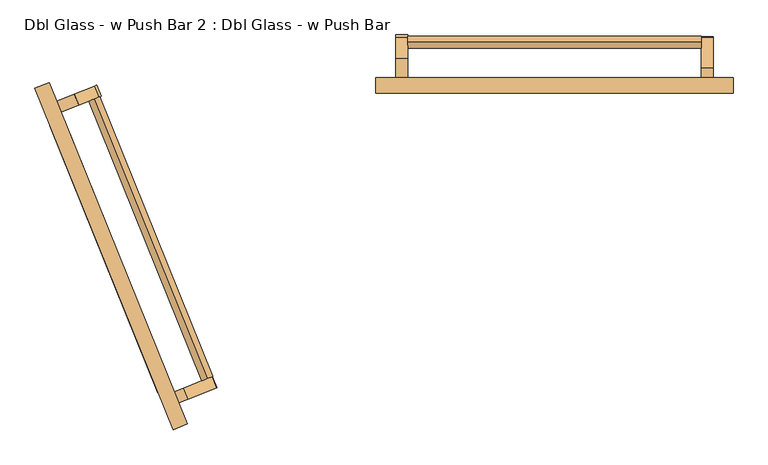
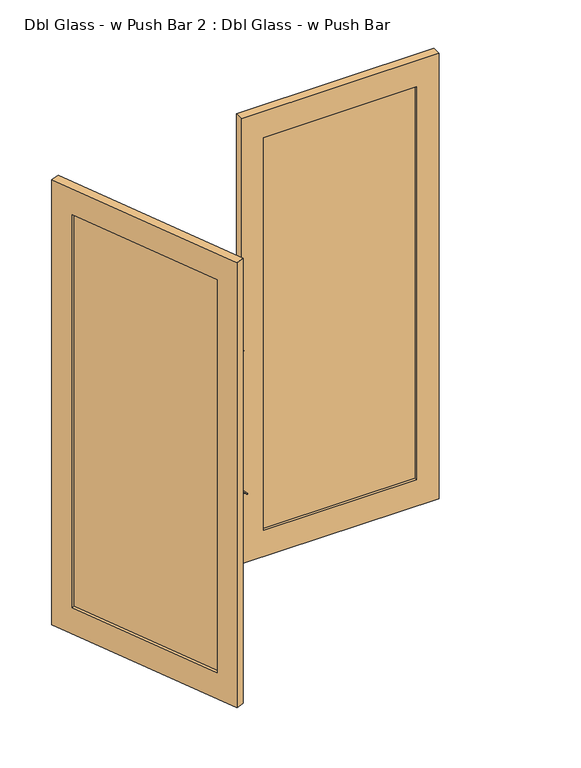
"""IFC4 building model written with IfcOpenShell, lengths in millimetres: door geometry, Dbl Glass - w Push Bar 2 : Dbl Glass - w Push Bar."""

import ifcopenshell
import ifcopenshell.guid

model = None  # the IFC model being written
_history = None  # IfcOwnerHistory: only IFC2X3 demands one
_inside = {}  # id of a spatial element -> (the spatial element, [elements in it])
_under = {}  # id of a project, library or spatial element -> (it, [spatial elements below it])
_declared = {}  # id of a project -> (the project, [libraries it declares])
_typed = {}  # id of a type object -> (the type object, [elements of that type])
_made_of = {}  # id of a material, layer set ... -> (it, [elements and type objects made of it])


def new_model(schema):
    """Start an empty IFC model of exactly this schema.

    Asked for "IFC4X3", IfcOpenShell would pick the latest addendum, in which some entities
    have other attributes; the version numbers below select the first issue.
    IFC2X3 requires an IfcOwnerHistory on every rooted entity: one is made here for all.
    """
    global model, _history
    if schema == "IFC4X3":
        model = ifcopenshell.file(schema_version=(4, 3, 0, 0))
    else:
        model = ifcopenshell.file(schema=schema)
    _inside.clear()
    _under.clear()
    _declared.clear()
    _typed.clear()
    _made_of.clear()
    _history = None
    if model.schema == "IFC2X3":
        org = make("IfcOrganization", Name="unknown")
        user = make(
            "IfcPersonAndOrganization",
            ThePerson=make("IfcPerson", FamilyName="unknown"),
            TheOrganization=org,
        )
        app = make(
            "IfcApplication",
            ApplicationDeveloper=org,
            Version="unknown",
            ApplicationFullName="unknown",
            ApplicationIdentifier="unknown",
        )
        _history = make(
            "IfcOwnerHistory",
            OwningUser=user,
            OwningApplication=app,
            ChangeAction="ADDED",
            CreationDate=0,
        )
    return model


def make(cls, **values):
    """One entity of the class cls with the attributes given. An attribute that is None is left unset."""
    return model.create_entity(
        cls, **{name: value for name, value in values.items() if value is not None}
    )


def rooted(cls, **values):
    """An entity with a GlobalId (a new one), such as an element, a storey or a relation."""
    return make(cls, GlobalId=ifcopenshell.guid.new(), OwnerHistory=_history, **values)


def si_unit(unit_type, name, prefix=None):
    """IfcSIUnit, for example si_unit("LENGTHUNIT", "METRE", prefix="MILLI")."""
    return make("IfcSIUnit", UnitType=unit_type, Prefix=prefix, Name=name)


def assignment(units):
    """IfcUnitAssignment: the units of a project."""
    return None if units is None else make("IfcUnitAssignment", Units=units)


def point(xyz):
    """IfcCartesianPoint."""
    return None if xyz is None else make("IfcCartesianPoint", Coordinates=xyz)


def direction(xyz):
    """IfcDirection."""
    return None if xyz is None else make("IfcDirection", DirectionRatios=xyz)


def frame(location, z_axis=None, x_axis=None):
    """IfcAxis2Placement3D, a coordinate frame: its origin and axes. An axis left out is left unset."""
    return make(
        "IfcAxis2Placement3D",
        Location=point(location),
        Axis=direction(z_axis),
        RefDirection=direction(x_axis),
    )


def frame_2d(location, x_axis=None):
    """IfcAxis2Placement2D, a coordinate frame in the plane: its origin and x axis."""
    return make(
        "IfcAxis2Placement2D", Location=point(location), RefDirection=direction(x_axis)
    )


def origin():
    """The frame at (0, 0, 0) with its axes left unset."""
    return frame((0.0, 0.0, 0.0))


def place(relative_to, where):
    """IfcLocalPlacement: puts the frame where relative to a parent placement (None: the world)."""
    return make(
        "IfcLocalPlacement", PlacementRelTo=relative_to, RelativePlacement=where
    )


def context(
    kind, dimensions, precision=None, world=None, true_north=None, identifier=None
):
    """IfcGeometricRepresentationContext, for example the 3D "Model" context."""
    return make(
        "IfcGeometricRepresentationContext",
        ContextIdentifier=identifier,
        ContextType=kind,
        CoordinateSpaceDimension=dimensions,
        Precision=precision,
        WorldCoordinateSystem=world,
        TrueNorth=true_north,
    )


def project(units=None, contexts=None):
    """IfcProject with its units and contexts."""
    return rooted(
        "IfcProject",
        Name="project",
        RepresentationContexts=contexts,
        UnitsInContext=assignment(units),
    )


def spatial(cls, under=None, at=None, **own):
    """A site, building, storey or space (cls), placed at a placement, below another one or the project."""
    s = rooted(cls, ObjectPlacement=at, **own)
    if under is not None:
        _under.setdefault(under.id(), (under, []))[1].append(s)
    return s


def polyline(points):
    """IfcPolyline through the points."""
    return make("IfcPolyline", Points=[point(p) for p in points])


def circle_curve(where, radius):
    """IfcCircle in the frame where."""
    return make("IfcCircle", Position=where, Radius=radius)


def trimmed(basis, trim1, trim2, sense, master):
    """IfcTrimmedCurve: the piece of a basis curve between two trims."""
    return make(
        "IfcTrimmedCurve",
        BasisCurve=basis,
        Trim1=trim1,
        Trim2=trim2,
        SenseAgreement=sense,
        MasterRepresentation=master,
    )


def segment(curve, same_sense, transition):
    """IfcCompositeCurveSegment."""
    return make(
        "IfcCompositeCurveSegment",
        Transition=transition,
        SameSense=same_sense,
        ParentCurve=curve,
    )


def composite_curve(segments, self_intersect=None):
    """IfcCompositeCurve: segments joined end to end."""
    return make("IfcCompositeCurve", Segments=segments, SelfIntersect=self_intersect)


def outline(outer, holes=None, kind="AREA"):
    """IfcArbitraryClosedProfileDef: a profile drawn as a closed curve; with holes, ...WithVoids."""
    if holes is None:
        return make("IfcArbitraryClosedProfileDef", ProfileType=kind, OuterCurve=outer)
    return make(
        "IfcArbitraryProfileDefWithVoids",
        ProfileType=kind,
        OuterCurve=outer,
        InnerCurves=holes,
    )


def extrude(swept, where, along, depth):
    """IfcExtrudedAreaSolid: the profile swept, set in the frame where, extruded along a direction by depth."""
    return make(
        "IfcExtrudedAreaSolid",
        SweptArea=swept,
        Position=where,
        ExtrudedDirection=direction(along),
        Depth=depth,
    )


def shape(context_of_items, identifier, shape_type, items):
    """IfcShapeRepresentation: the items that make up one representation, for example the "Body"."""
    return make(
        "IfcShapeRepresentation",
        ContextOfItems=context_of_items,
        RepresentationIdentifier=identifier,
        RepresentationType=shape_type,
        Items=items,
    )


def source(mapping_origin, context_of_items, identifier, shape_type, items):
    """IfcRepresentationMap: a shape defined once, which mapped items show again and again."""
    return make(
        "IfcRepresentationMap",
        MappingOrigin=mapping_origin,
        MappedRepresentation=shape(context_of_items, identifier, shape_type, items),
    )


def transform(
    local_origin,
    x_axis=None,
    y_axis=None,
    z_axis=None,
    scale=None,
    scale2=None,
    scale3=None,
    uniform=True,
):
    """IfcCartesianTransformationOperator3D, or its non-uniform kind. x_axis, y_axis, z_axis: its Axis1, 2, 3."""
    if uniform:
        return make(
            "IfcCartesianTransformationOperator3D",
            Axis1=direction(x_axis),
            Axis2=direction(y_axis),
            LocalOrigin=point(local_origin),
            Scale=scale,
            Axis3=direction(z_axis),
        )
    return make(
        "IfcCartesianTransformationOperator3DnonUniform",
        Axis1=direction(x_axis),
        Axis2=direction(y_axis),
        LocalOrigin=point(local_origin),
        Scale=scale,
        Axis3=direction(z_axis),
        Scale2=scale2,
        Scale3=scale3,
    )


def mapped(mapping_source, mapping_target):
    """IfcMappedItem: shows the shape of a source again, moved by a transform."""
    return make(
        "IfcMappedItem", MappingSource=mapping_source, MappingTarget=mapping_target
    )


def made_of(thing, what):
    """Note that an element or type object is made of a material, layer set ...; save() writes the relation."""
    if what is not None:
        _made_of.setdefault(what.id(), (what, []))[1].append(thing)
    return thing


def element(
    cls,
    number,
    at=None,
    inside=None,
    cuts=None,
    type_object=None,
    material=None,
    context=None,
    identifier="Body",
    shape_type=None,
    held_by="IfcProductDefinitionShape",
    body=None,
    shapes=None,
    **own,
):
    """One element of the class cls, such as IfcWall. Its Tag is "e" and its number.

    at: its placement. inside: the storey or other place that contains it. cuts: it is an
    opening in that element (IfcRelVoidsElement). A single representation is given by context,
    identifier, shape_type and body (its items); several are given by shapes. held_by: the class
    of the entity that holds the representations. save() writes the other relations.
    """
    e = rooted(cls, Tag="e%d" % number, ObjectPlacement=at, **own)
    if body is not None:
        shapes = [shape(context, identifier, shape_type, body)]
    if shapes is not None:
        e.Representation = make(held_by, Representations=shapes)
    if inside is not None:
        _inside.setdefault(inside.id(), (inside, []))[1].append(e)
    if cuts is not None:
        rooted(
            "IfcRelVoidsElement", RelatingBuildingElement=cuts, RelatedOpeningElement=e
        )
    if type_object is not None:
        _typed.setdefault(type_object.id(), (type_object, []))[1].append(e)
    return made_of(e, material)


def aggregate(whole, parts):
    """IfcRelAggregates: a whole, such as a stair, and the parts it consists of."""
    return rooted("IfcRelAggregates", RelatingObject=whole, RelatedObjects=parts)


def save(model, path):
    """Write the relations noted so far, then the file.

    IfcRelAggregates (storeys below a building ...), IfcRelContainedInSpatialStructure (elements
    in a storey), IfcRelDefinesByType, IfcRelAssociatesMaterial and IfcRelDeclares: one each for
    every whole, place, type object, material and project.
    """
    for whole, parts in _under.values():
        aggregate(whole, parts)
    for where, things in _inside.values():
        rooted(
            "IfcRelContainedInSpatialStructure",
            RelatedElements=things,
            RelatingStructure=where,
        )
    for kind, things in _typed.values():
        rooted("IfcRelDefinesByType", RelatedObjects=things, RelatingType=kind)
    for what, things in _made_of.values():
        rooted("IfcRelAssociatesMaterial", RelatedObjects=things, RelatingMaterial=what)
    for by, libraries in _declared.values():
        rooted("IfcRelDeclares", RelatingContext=by, RelatedDefinitions=libraries)
    model.write(path)


def dbl_glass_w_push_bar_2_dbl_glass_w_push_bar_dfafdb44(model_context):
    return source(origin(), model_context, "Body", "SweptSolid", [
        extrude(outline(composite_curve([segment(trimmed(circle_curve(frame_2d((65.0203019, 954.5721086)), 15.0), [point((65.0203019, 969.5721086))], [point((65.0203019, 939.5721086))], False, "CARTESIAN"), True, "CONTINUOUS"), segment(trimmed(circle_curve(frame_2d((65.0203019, 954.5721086)), 15.0), [point((65.0203019, 939.5721086))], [point((65.0203019, 969.5721086))], False, "CARTESIAN"), True, "CONTINUOUS")], self_intersect=False)), frame((80.0, 0.0, 0.0), z_axis=(1.0, 0.0, 0.0), x_axis=(0.0, 1.0, 0.0)), (0.0, 0.0, 1.0), 731.0),
        extrude(outline(composite_curve([segment(polyline([(-0.1563269, 1000.0), (77.6459332, 922.19774)]), True, "CONTINUOUS"), segment(trimmed(circle_curve(frame_2d((75.7878695, 920.3396763)), 2.6276989), [point((77.6459332, 922.19774))], [point((73.9298058, 918.4816126))], False, "CARTESIAN"), True, "CONTINUOUS"), segment(polyline([(73.9298058, 918.4816126), (57.4114184, 935.0), (-24.035259, 935.0), (-24.035259, 1000.0), (-0.1563269, 1000.0)]), True, "CONTINUOUS")], self_intersect=False)), frame((811.0, 0.0, 0.0), z_axis=(1.0, 0.0, 0.0), x_axis=(0.0, 1.0, 0.0)), (0.0, 0.0, 1.0), 30.0),
        extrude(outline(composite_curve([segment(polyline([(23.375226, 1000.0), (77.6459332, 945.7292928)]), True, "CONTINUOUS"), segment(trimmed(circle_curve(frame_2d((65.0203019, 933.1036615)), 17.8553391), [point((77.6459332, 945.7292928))], [point((52.3946705, 920.4780301))], False, "CARTESIAN"), True, "CONTINUOUS"), segment(polyline([(52.3946705, 920.4780301), (37.8727007, 935.0), (-24.035259, 935.0), (-24.035259, 1000.0), (23.375226, 1000.0)]), True, "CONTINUOUS")], self_intersect=False)), frame((50.0, 0.0, 0.0), z_axis=(1.0, 0.0, 0.0), x_axis=(0.0, 1.0, 0.0)), (0.0, 0.0, 1.0), 30.0),
        extrude(outline(composite_curve([segment(trimmed(circle_curve(frame_2d((0.0, 15.0)), 15.0), [point((0.0, 30.0))], [point((0.0, 0.0))], False, "CARTESIAN"), True, "CONTINUOUS"), segment(trimmed(circle_curve(frame_2d((0.0, 15.0)), 15.0), [point((0.0, 0.0))], [point((0.0, 30.0))], False, "CARTESIAN"), True, "CONTINUOUS")], self_intersect=False)), frame((-419.6508941, -774.4258968, 939.5721086), z_axis=(-0.37460659341591906, 0.9271838545667846, 0.0), x_axis=(-0.9271838545667846, -0.37460659341591906, 0.0)), (0.0, 0.0, 1.0), 752.3041635),
        extrude(outline(composite_curve([segment(polyline([(23.8789322, 0.0), (0.0, 0.0), (0.0, 65.0), (81.4466774, 65.0), (97.9650649, 81.5183874)]), True, "CONTINUOUS"), segment(trimmed(circle_curve(frame_2d((99.8231285, 79.6603237)), 2.6276989), [point((97.9650649, 81.5183874))], [point((101.6811923, 77.80226))], False, "CARTESIAN"), True, "CONTINUOUS"), segment(polyline([(101.6811923, 77.80226), (23.8789322, 0.0)]), True, "CONTINUOUS")], self_intersect=False)), frame((-490.9835746, -835.6022127, 1000.0), z_axis=(-0.37460659341591906, 0.9271838545667846, 0.0), x_axis=(0.9271838545667846, 0.37460659341591906, 0.0)), (0.0, 0.0, 1.0), 30.0),
        extrude(outline(composite_curve([segment(polyline([(47.4104851, 0.0), (0.0, 0.0), (0.0, 65.0), (61.9079597, 65.0), (76.4299296, 79.5219699)]), True, "CONTINUOUS"), segment(trimmed(circle_curve(frame_2d((89.055561, 66.8963385)), 17.8553391), [point((76.4299296, 79.5219699))], [point((101.6811923, 54.2707072))], False, "CARTESIAN"), True, "CONTINUOUS"), segment(polyline([(101.6811923, 54.2707072), (47.4104851, 0.0)]), True, "CONTINUOUS")], self_intersect=False)), frame((-784.0398723, -110.262423, 1000.0), z_axis=(-0.37460659341591906, 0.9271838545667846, 0.0), x_axis=(0.9271838545667846, 0.37460659341591906, 0.0)), (0.0, 0.0, 1.0), 30.0),
        extrude(outline(polyline([(0.0, 0.0), (-2125.0, 0.0), (-2125.0, 919.2412593), (0.0, 919.2412593), (0.0, 0.0)]), holes=[polyline([(-125.0, 100.0000001), (-125.0, 819.2412594), (-2000.0, 819.2412594), (-2000.0, 100.0000001), (-125.0, 100.0000001)])]), frame((-849.7454002, -50.5264, 2125.0), z_axis=(0.9271838545667834, 0.37460659341592206, 0.0), x_axis=(0.0, 0.0, 1.0)), (0.0, 0.0, 1.0), 38.5435966),
        extrude(outline(polyline([(2125.0, 0.0), (0.0, 0.0), (0.0, 891.0), (2125.0, 891.0), (2125.0, 0.0)]), holes=[polyline([(2000.0, 100.0), (2000.0, 791.0), (125.0, 791.0), (125.0, 100.0), (2000.0, 100.0)])]), frame((0.0, -62.5788556, 0.0), z_axis=(0.0, 1.0, 0.0), x_axis=(0.0, 0.0, 1.0)), (0.0, 0.0, 1.0), 38.5435966),
        extrude(outline(polyline([(-520.0631047, -800.9062673), (-531.189311, -805.4015464), (-800.621829, -138.5326632), (-789.4956227, -134.0373841), (-520.0631047, -800.9062673)])), frame((0.0, 0.0, 125.0), z_axis=(0.0, 0.0, 1.0), x_axis=(1.0, 0.0, 0.0)), (0.0, 0.0, 1.0), 1875.0),
        extrude(outline(polyline([(791.0, -38.0), (791.0, -50.0), (100.0, -50.0), (100.0, -38.0), (791.0, -38.0)])), frame((0.0, 0.0, 125.0), z_axis=(0.0, 0.0, 1.0), x_axis=(1.0, 0.0, 0.0)), (0.0, 0.0, 1.0), 1875.0),
    ])


if __name__ == "__main__":
    model = new_model("IFC4")
    model_context = context("Model", 3, world=origin())
    ifc_project = project(units=[si_unit("LENGTHUNIT", "METRE", prefix="MILLI")], contexts=[model_context])
    site = spatial("IfcSite", under=ifc_project)
    building = spatial("IfcBuilding", under=site)
    placement = place(None, origin())
    dbl_glass_w_push_bar_2_dbl_glass_w_push_bar_shape = dbl_glass_w_push_bar_2_dbl_glass_w_push_bar_dfafdb44(model_context)
    element("IfcDoor", 1, ObjectType="Dbl Glass - w Push Bar 2 : Dbl Glass - w Push Bar", at=placement, inside=building, context=model_context, shape_type="MappedRepresentation", body=[
        mapped(dbl_glass_w_push_bar_2_dbl_glass_w_push_bar_shape, transform((0.0, 0.0, 0.0), x_axis=(1.0, 0.0, 0.0), y_axis=(0.0, 1.0, 0.0), z_axis=(0.0, 0.0, 1.0))),
    ])
    save(model, "model.ifc")

# Revit data of these elements
# Type "Dbl Glass - w Push Bar 2 : Dbl Glass - w Push Bar"
#   Type Mark = "68"
#   Description = "Curtain Wall Door"
#   Construction Type Id = "GSP4R"
#   Analytic Construction = "1/8 in Pilkington single glazing"
#   Visual Light Transmittance = 0.9
#   TopRail = 125 mm
#   Thermal Resistance (R) = 0.271106 (m²·K)/W
#   Solar Heat Gain Coefficient = 0.78
#   Offset = 50 mm
#   MuntinRail = 100 mm
#   LockRail = 100 mm
#   Heat Transfer Coefficient (U) = 3.6886 W/(m²·K)
#   Handle Z Distance = 1000 mm
#   Handle X Offset = 65 mm
#   Glass Thickness = 12 mm
#   BottomRail = 125 mm
#   Define Thermal Properties by = 1
#   Material Ironmongery = Metal - Aluminum
#   Material Door = Metal - Aluminum
#   Material Glass = Glass
#   Function = (empty or 0)
# Element 1 (IfcDoor, "Dbl Glass - w Push Bar 2 : Dbl Glass - w Push Bar")
#   Materials on its faces: "Metal - Aluminum", "Glass"
# Materials
#   "Metal - Aluminum": class "Metal", colour RGB 247 247 247, transparency 0
#   "Glass": class "Glass", colour RGB 0 128 192, transparency 0.9, Description = "Soda Lime Glass", Cost = 0
